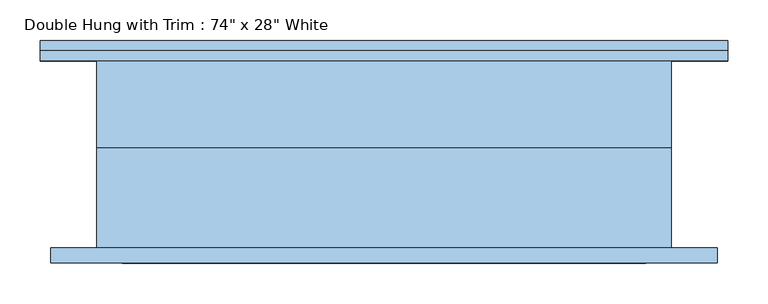
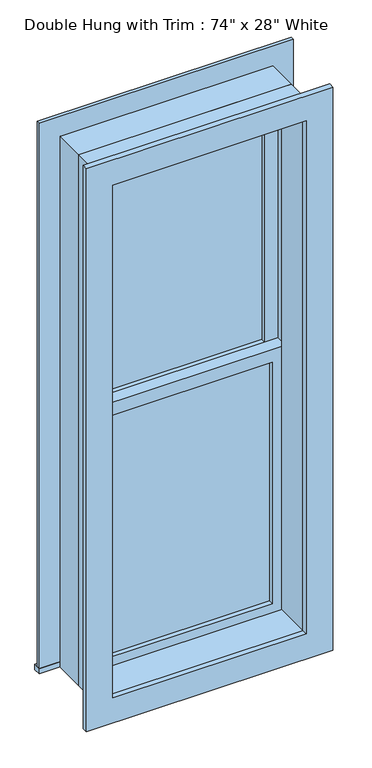
"""IFC4 building model written with IfcOpenShell, lengths in millimetres: window geometry."""

from ifc_helpers import new_model, si_unit, frame, origin, place, context, project, spatial, polyline, outline, extrude, source, transform, mapped, element, save


def window_28ccb7d3(model_context):
    return source(origin(), model_context, "Body", "SweptSolid", [
        extrude(outline(polyline([(-292.1, 36.5125008), (292.1, 36.5125008), (292.1, 23.8125008), (-292.1, 23.8125008), (-292.1, 36.5125008)])), frame((0.0, 0.0, 571.5), z_axis=(0.0, 0.0, 1.0), x_axis=(1.0, 0.0, 0.0)), (0.0, 0.0, 1.0), 854.075),
        extrude(outline(polyline([(1470.025, -336.55), (527.05, -336.55), (527.05, 336.55), (1470.025, 336.55), (1470.025, -336.55)]), holes=[polyline([(1425.575, -292.1), (1425.575, 292.1), (571.5, 292.1), (571.5, -292.1), (1425.575, -292.1)])]), frame((0.0, 7.9375008, 0.0), z_axis=(0.0, 1.0, 0.0), x_axis=(0.0, 0.0, 1.0)), (0.0, 0.0, 1.0), 44.45),
        extrude(outline(polyline([(-425.45, 141.2875008), (425.45, 141.2875008), (425.45, 115.8875008), (-425.45, 115.8875008), (-425.45, 141.2875008)])), frame((0.0, 0.0, 508.0), z_axis=(0.0, 0.0, 1.0), x_axis=(1.0, 0.0, 0.0)), (0.0, 0.0, 1.0), 19.05),
        extrude(outline(polyline([(2368.55, -336.55), (2368.55, 336.55), (527.05, 336.55), (527.05, 425.45), (2457.45, 425.45), (2457.45, -425.45), (527.05, -425.45), (527.05, -336.55), (2368.55, -336.55)])), frame((0.0, 115.8875008, 0.0), z_axis=(0.0, 1.0, 0.0), x_axis=(0.0, 0.0, 1.0)), (0.0, 0.0, 1.0), 12.7),
        extrude(outline(polyline([(2444.75, 412.75), (2444.75, -412.75), (450.85, -412.75), (450.85, 412.75), (2444.75, 412.75)]), holes=[polyline([(2355.85, 323.85), (539.75, 323.85), (539.75, -323.85), (2355.85, -323.85), (2355.85, 323.85)])]), frame((0.0, -134.9375008, 0.0), z_axis=(0.0, 1.0, 0.0), x_axis=(0.0, 0.0, 1.0)), (0.0, 0.0, 1.0), 19.05),
        extrude(outline(polyline([(292.1, 68.2625008), (-292.1, 68.2625008), (-292.1, 80.9625008), (292.1, 80.9625008), (292.1, 68.2625008)])), frame((0.0, 0.0, 1470.025), z_axis=(0.0, 0.0, 1.0), x_axis=(1.0, 0.0, 0.0)), (0.0, 0.0, 1.0), 854.075),
        extrude(outline(polyline([(2368.55, -336.55), (1425.575, -336.55), (1425.575, 336.55), (2368.55, 336.55), (2368.55, -336.55)]), holes=[polyline([(2324.1, -292.1), (2324.1, 292.1), (1470.025, 292.1), (1470.025, -292.1), (2324.1, -292.1)])]), frame((0.0, 52.3875008, 0.0), z_axis=(0.0, 1.0, 0.0), x_axis=(0.0, 0.0, 1.0)), (0.0, 0.0, 1.0), 44.45),
        extrude(outline(polyline([(2387.6, -355.6), (508.0, -355.6), (508.0, 355.6), (2387.6, 355.6), (2387.6, -355.6)]), holes=[polyline([(2355.85, -323.85), (2355.85, 323.85), (539.75, 323.85), (539.75, -323.85), (2355.85, -323.85)])]), frame((0.0, -115.8875008, 0.0), z_axis=(0.0, 1.0, 0.0), x_axis=(0.0, 0.0, 1.0)), (0.0, 0.0, 1.0), 123.8250015),
        extrude(outline(polyline([(2387.6, 355.6), (2387.6, -355.6), (508.0, -355.6), (508.0, 355.6), (2387.6, 355.6)]), holes=[polyline([(2368.55, 336.55), (527.05, 336.55), (527.05, -336.55), (2368.55, -336.55), (2368.55, 336.55)])]), frame((0.0, 7.9375008, 0.0), z_axis=(0.0, 1.0, 0.0), x_axis=(0.0, 0.0, 1.0)), (0.0, 0.0, 1.0), 107.95),
    ])


if __name__ == "__main__":
    model = new_model("IFC4")
    model_context = context("Model", 3, world=origin())
    ifc_project = project(units=[si_unit("LENGTHUNIT", "METRE", prefix="MILLI")], contexts=[model_context])
    site = spatial("IfcSite", under=ifc_project)
    building = spatial("IfcBuilding", under=site)
    placement = place(None, origin())
    window_shape = window_28ccb7d3(model_context)
    element("IfcWindow", 1, ObjectType="Double Hung with Trim : 74\" x 28\" White", at=placement, inside=building, context=model_context, shape_type="MappedRepresentation", body=[
        mapped(window_shape, transform((0.0, 0.0, 0.0), x_axis=(1.0, 0.0, 0.0), y_axis=(0.0, 1.0, 0.0), z_axis=(0.0, 0.0, 1.0))),
    ])
    save(model, "model.ifc")

# Revit data of these elements
# Type "Double Hung with Trim : 74\" x 28\" White"
#   Type Mark = "78"
#   Construction Type Id = "GSP4R"
#   Assembly Code = "B2020100"
#   Analytic Construction = "1/8 in Pilkington single glazing"
#   Visual Light Transmittance = 0.9
#   Solar Heat Gain Coefficient = 0.78
#   Heat Transfer Coefficient (U) = 3.6886 W/(m²·K)
#   Height = 6' - 2"
#   Default Sill Height = 1' - 8"
#   Trim Projection - Ext. = 0' - 0 1/2"
#   Trim Projection - Int. = 0' - 0 3/4"
#   Trim Width - Exterior = 0' - 3 1/2"
#   Trim Width - Interior = 0' - 3 1/2"
#   Width = 2' - 4"
#   Window Inset = 0' - 0 3/4"
#   COBie.Type = no
#   Glass Pane Material = Glass
#   Sash Material = Sash - White
#   Trim Exterior Material = Trim - White
#   Trim Interior Material = Trim - White
#   Wall Closure = (empty or 0)
# Element 1 (IfcWindow, "Double Hung with Trim : 74\" x 28\" White")
#   Materials on its faces: "Sash - White", "Trim - White", "Glass"
# Materials
#   "Glass": class "Glass", colour RGB 0 128 192, transparency 0.75, Description = "Soda Lime Glass", Cost = 0
#   "Sash - White": class "Wood", colour RGB 255 255 255, transparency 0, Cost = 0
#   "Trim - White": class "Wood", colour RGB 255 255 255, transparency 0, Cost = 0
